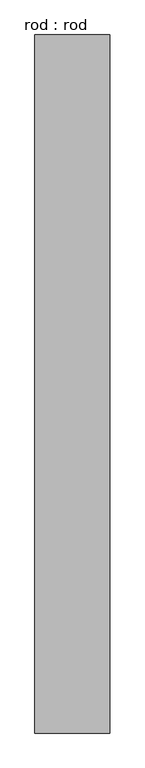
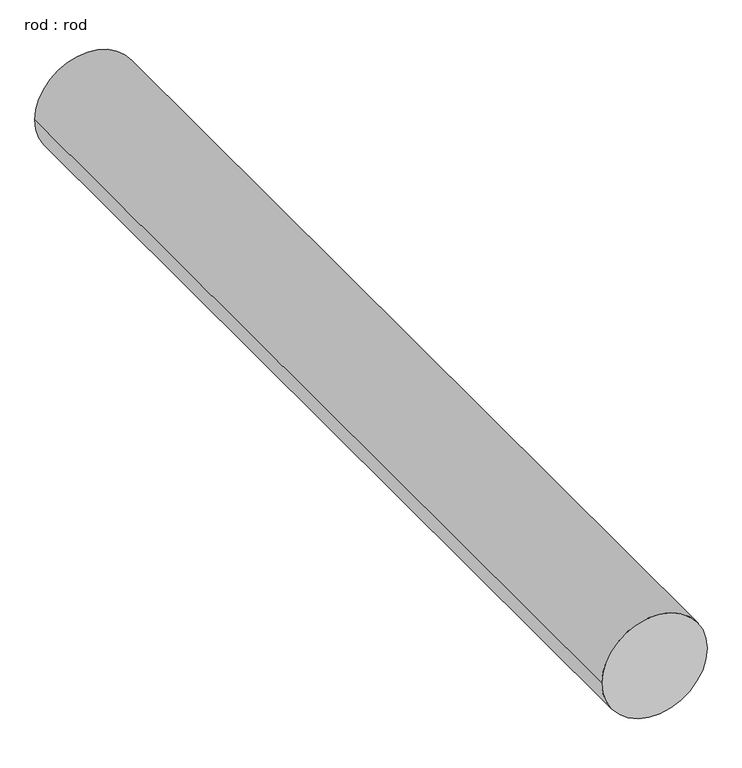
"""IFC4 building model written with IfcOpenShell, lengths in millimetres: proxy geometry, rod : rod."""

import ifcopenshell
import ifcopenshell.guid

model = None  # the IFC model being written
_history = None  # IfcOwnerHistory: only IFC2X3 demands one
_inside = {}  # id of a spatial element -> (the spatial element, [elements in it])
_under = {}  # id of a project, library or spatial element -> (it, [spatial elements below it])
_declared = {}  # id of a project -> (the project, [libraries it declares])
_typed = {}  # id of a type object -> (the type object, [elements of that type])
_made_of = {}  # id of a material, layer set ... -> (it, [elements and type objects made of it])


def new_model(schema):
    """Start an empty IFC model of exactly this schema.

    Asked for "IFC4X3", IfcOpenShell would pick the latest addendum, in which some entities
    have other attributes; the version numbers below select the first issue.
    IFC2X3 requires an IfcOwnerHistory on every rooted entity: one is made here for all.
    """
    global model, _history
    if schema == "IFC4X3":
        model = ifcopenshell.file(schema_version=(4, 3, 0, 0))
    else:
        model = ifcopenshell.file(schema=schema)
    _inside.clear()
    _under.clear()
    _declared.clear()
    _typed.clear()
    _made_of.clear()
    _history = None
    if model.schema == "IFC2X3":
        org = make("IfcOrganization", Name="unknown")
        user = make(
            "IfcPersonAndOrganization",
            ThePerson=make("IfcPerson", FamilyName="unknown"),
            TheOrganization=org,
        )
        app = make(
            "IfcApplication",
            ApplicationDeveloper=org,
            Version="unknown",
            ApplicationFullName="unknown",
            ApplicationIdentifier="unknown",
        )
        _history = make(
            "IfcOwnerHistory",
            OwningUser=user,
            OwningApplication=app,
            ChangeAction="ADDED",
            CreationDate=0,
        )
    return model


def make(cls, **values):
    """One entity of the class cls with the attributes given. An attribute that is None is left unset."""
    return model.create_entity(
        cls, **{name: value for name, value in values.items() if value is not None}
    )


def rooted(cls, **values):
    """An entity with a GlobalId (a new one), such as an element, a storey or a relation."""
    return make(cls, GlobalId=ifcopenshell.guid.new(), OwnerHistory=_history, **values)


def si_unit(unit_type, name, prefix=None):
    """IfcSIUnit, for example si_unit("LENGTHUNIT", "METRE", prefix="MILLI")."""
    return make("IfcSIUnit", UnitType=unit_type, Prefix=prefix, Name=name)


def assignment(units):
    """IfcUnitAssignment: the units of a project."""
    return None if units is None else make("IfcUnitAssignment", Units=units)


def point(xyz):
    """IfcCartesianPoint."""
    return None if xyz is None else make("IfcCartesianPoint", Coordinates=xyz)


def direction(xyz):
    """IfcDirection."""
    return None if xyz is None else make("IfcDirection", DirectionRatios=xyz)


def frame(location, z_axis=None, x_axis=None):
    """IfcAxis2Placement3D, a coordinate frame: its origin and axes. An axis left out is left unset."""
    return make(
        "IfcAxis2Placement3D",
        Location=point(location),
        Axis=direction(z_axis),
        RefDirection=direction(x_axis),
    )


def frame_2d(location, x_axis=None):
    """IfcAxis2Placement2D, a coordinate frame in the plane: its origin and x axis."""
    return make(
        "IfcAxis2Placement2D", Location=point(location), RefDirection=direction(x_axis)
    )


def origin():
    """The frame at (0, 0, 0) with its axes left unset."""
    return frame((0.0, 0.0, 0.0))


def place(relative_to, where):
    """IfcLocalPlacement: puts the frame where relative to a parent placement (None: the world)."""
    return make(
        "IfcLocalPlacement", PlacementRelTo=relative_to, RelativePlacement=where
    )


def context(
    kind, dimensions, precision=None, world=None, true_north=None, identifier=None
):
    """IfcGeometricRepresentationContext, for example the 3D "Model" context."""
    return make(
        "IfcGeometricRepresentationContext",
        ContextIdentifier=identifier,
        ContextType=kind,
        CoordinateSpaceDimension=dimensions,
        Precision=precision,
        WorldCoordinateSystem=world,
        TrueNorth=true_north,
    )


def project(units=None, contexts=None):
    """IfcProject with its units and contexts."""
    return rooted(
        "IfcProject",
        Name="project",
        RepresentationContexts=contexts,
        UnitsInContext=assignment(units),
    )


def spatial(cls, under=None, at=None, **own):
    """A site, building, storey or space (cls), placed at a placement, below another one or the project."""
    s = rooted(cls, ObjectPlacement=at, **own)
    if under is not None:
        _under.setdefault(under.id(), (under, []))[1].append(s)
    return s


def circle_curve(where, radius):
    """IfcCircle in the frame where."""
    return make("IfcCircle", Position=where, Radius=radius)


def trimmed(basis, trim1, trim2, sense, master):
    """IfcTrimmedCurve: the piece of a basis curve between two trims."""
    return make(
        "IfcTrimmedCurve",
        BasisCurve=basis,
        Trim1=trim1,
        Trim2=trim2,
        SenseAgreement=sense,
        MasterRepresentation=master,
    )


def segment(curve, same_sense, transition):
    """IfcCompositeCurveSegment."""
    return make(
        "IfcCompositeCurveSegment",
        Transition=transition,
        SameSense=same_sense,
        ParentCurve=curve,
    )


def composite_curve(segments, self_intersect=None):
    """IfcCompositeCurve: segments joined end to end."""
    return make("IfcCompositeCurve", Segments=segments, SelfIntersect=self_intersect)


def outline(outer, holes=None, kind="AREA"):
    """IfcArbitraryClosedProfileDef: a profile drawn as a closed curve; with holes, ...WithVoids."""
    if holes is None:
        return make("IfcArbitraryClosedProfileDef", ProfileType=kind, OuterCurve=outer)
    return make(
        "IfcArbitraryProfileDefWithVoids",
        ProfileType=kind,
        OuterCurve=outer,
        InnerCurves=holes,
    )


def extrude(swept, where, along, depth):
    """IfcExtrudedAreaSolid: the profile swept, set in the frame where, extruded along a direction by depth."""
    return make(
        "IfcExtrudedAreaSolid",
        SweptArea=swept,
        Position=where,
        ExtrudedDirection=direction(along),
        Depth=depth,
    )


def shape(context_of_items, identifier, shape_type, items):
    """IfcShapeRepresentation: the items that make up one representation, for example the "Body"."""
    return make(
        "IfcShapeRepresentation",
        ContextOfItems=context_of_items,
        RepresentationIdentifier=identifier,
        RepresentationType=shape_type,
        Items=items,
    )


def source(mapping_origin, context_of_items, identifier, shape_type, items):
    """IfcRepresentationMap: a shape defined once, which mapped items show again and again."""
    return make(
        "IfcRepresentationMap",
        MappingOrigin=mapping_origin,
        MappedRepresentation=shape(context_of_items, identifier, shape_type, items),
    )


def transform(
    local_origin,
    x_axis=None,
    y_axis=None,
    z_axis=None,
    scale=None,
    scale2=None,
    scale3=None,
    uniform=True,
):
    """IfcCartesianTransformationOperator3D, or its non-uniform kind. x_axis, y_axis, z_axis: its Axis1, 2, 3."""
    if uniform:
        return make(
            "IfcCartesianTransformationOperator3D",
            Axis1=direction(x_axis),
            Axis2=direction(y_axis),
            LocalOrigin=point(local_origin),
            Scale=scale,
            Axis3=direction(z_axis),
        )
    return make(
        "IfcCartesianTransformationOperator3DnonUniform",
        Axis1=direction(x_axis),
        Axis2=direction(y_axis),
        LocalOrigin=point(local_origin),
        Scale=scale,
        Axis3=direction(z_axis),
        Scale2=scale2,
        Scale3=scale3,
    )


def mapped(mapping_source, mapping_target):
    """IfcMappedItem: shows the shape of a source again, moved by a transform."""
    return make(
        "IfcMappedItem", MappingSource=mapping_source, MappingTarget=mapping_target
    )


def made_of(thing, what):
    """Note that an element or type object is made of a material, layer set ...; save() writes the relation."""
    if what is not None:
        _made_of.setdefault(what.id(), (what, []))[1].append(thing)
    return thing


def element(
    cls,
    number,
    at=None,
    inside=None,
    cuts=None,
    type_object=None,
    material=None,
    context=None,
    identifier="Body",
    shape_type=None,
    held_by="IfcProductDefinitionShape",
    body=None,
    shapes=None,
    **own,
):
    """One element of the class cls, such as IfcWall. Its Tag is "e" and its number.

    at: its placement. inside: the storey or other place that contains it. cuts: it is an
    opening in that element (IfcRelVoidsElement). A single representation is given by context,
    identifier, shape_type and body (its items); several are given by shapes. held_by: the class
    of the entity that holds the representations. save() writes the other relations.
    """
    e = rooted(cls, Tag="e%d" % number, ObjectPlacement=at, **own)
    if body is not None:
        shapes = [shape(context, identifier, shape_type, body)]
    if shapes is not None:
        e.Representation = make(held_by, Representations=shapes)
    if inside is not None:
        _inside.setdefault(inside.id(), (inside, []))[1].append(e)
    if cuts is not None:
        rooted(
            "IfcRelVoidsElement", RelatingBuildingElement=cuts, RelatedOpeningElement=e
        )
    if type_object is not None:
        _typed.setdefault(type_object.id(), (type_object, []))[1].append(e)
    return made_of(e, material)


def aggregate(whole, parts):
    """IfcRelAggregates: a whole, such as a stair, and the parts it consists of."""
    return rooted("IfcRelAggregates", RelatingObject=whole, RelatedObjects=parts)


def save(model, path):
    """Write the relations noted so far, then the file.

    IfcRelAggregates (storeys below a building ...), IfcRelContainedInSpatialStructure (elements
    in a storey), IfcRelDefinesByType, IfcRelAssociatesMaterial and IfcRelDeclares: one each for
    every whole, place, type object, material and project.
    """
    for whole, parts in _under.values():
        aggregate(whole, parts)
    for where, things in _inside.values():
        rooted(
            "IfcRelContainedInSpatialStructure",
            RelatedElements=things,
            RelatingStructure=where,
        )
    for kind, things in _typed.values():
        rooted("IfcRelDefinesByType", RelatedObjects=things, RelatingType=kind)
    for what, things in _made_of.values():
        rooted("IfcRelAssociatesMaterial", RelatedObjects=things, RelatingMaterial=what)
    for by, libraries in _declared.values():
        rooted("IfcRelDeclares", RelatingContext=by, RelatedDefinitions=libraries)
    model.write(path)


def rod_rod_e1cbed2a(model_context):
    return source(origin(), model_context, "Body", "SweptSolid", [
        extrude(outline(composite_curve([segment(trimmed(circle_curve(frame_2d((0.0108462, 0.0)), 200.0), [point((0.0108462, 200.0))], [point((0.0108462, -200.0))], False, "CARTESIAN"), True, "CONTINUOUS"), segment(trimmed(circle_curve(frame_2d((0.0108462, 0.0)), 200.0), [point((0.0108462, -200.0))], [point((0.0108462, 200.0))], False, "CARTESIAN"), True, "CONTINUOUS")], self_intersect=False)), frame((0.0, 2230.5373658, 0.0), z_axis=(0.0, 1.0, 0.0), x_axis=(0.0, 0.0, 1.0)), (0.0, 0.0, 1.0), 3724.3824992),
    ])


if __name__ == "__main__":
    model = new_model("IFC4")
    model_context = context("Model", 3, world=origin())
    ifc_project = project(units=[si_unit("LENGTHUNIT", "METRE", prefix="MILLI")], contexts=[model_context])
    site = spatial("IfcSite", under=ifc_project)
    building = spatial("IfcBuilding", under=site)
    placement = place(None, origin())
    rod_rod_shape = rod_rod_e1cbed2a(model_context)
    element("IfcBuildingElementProxy", 1, Name="rod : rod", ObjectType="rod : rod", at=placement, inside=building, context=model_context, shape_type="MappedRepresentation", body=[
        mapped(rod_rod_shape, transform((0.0, 0.0, 0.0), x_axis=(1.0, 0.0, 0.0), y_axis=(0.0, 1.0, 0.0), z_axis=(0.0, 0.0, 1.0))),
    ])
    save(model, "model.ifc")

# Revit data of these elements
# Type "rod : rod"
#   Default Elevation = 0
